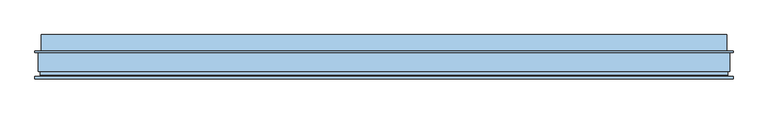
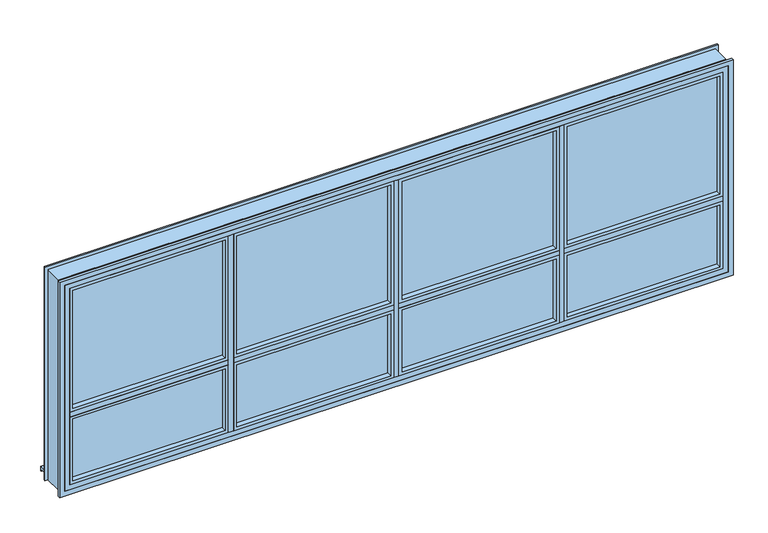
"""IFC4 building model written with IfcOpenShell, lengths in millimetres: window geometry, K-LINE ENSEMBLE COMPOSE NEUF KLT-8Z-4H2V : WD531_K-LINE ENSEMBLE COMPOSE NEUF KLT-8Z-4H2V."""

from ifc_helpers import new_model, si_unit, frame, origin, place, context, project, spatial, polyline, outline, extrude, faceted_brep, source, transform, mapped, element, save


def window_16f5b6b2(model_context):
    return source(origin(), model_context, "Body", "SolidModel", [
        extrude(outline(polyline([(-18.0, -155.0), (-18.0, -179.0), (-882.0, -179.0), (-882.0, -155.0), (-18.0, -155.0)])), frame((0.0, 0.0, 850.5), z_axis=(0.0, 0.0, 1.0), x_axis=(1.0, 0.0, 0.0)), (0.0, 0.0, 1.0), 381.5),
        extrude(outline(polyline([(1236.0, -14.0), (1236.0, -886.0), (846.5, -886.0), (846.5, -14.0), (1236.0, -14.0)]), holes=[polyline([(863.5, -31.0), (863.5, -869.0), (1219.0, -869.0), (1219.0, -31.0), (863.5, -31.0)])]), frame((0.0, -207.5, 0.0), z_axis=(0.0, 1.0, 0.0), x_axis=(0.0, 0.0, 1.0)), (0.0, 0.0, 1.0), 28.5),
        extrude(outline(polyline([(-18.0, -155.0), (-18.0, -179.0), (-882.0, -179.0), (-882.0, -155.0), (-18.0, -155.0)])), frame((0.0, 0.0, 1268.0), z_axis=(0.0, 0.0, 1.0), x_axis=(1.0, 0.0, 0.0)), (0.0, 0.0, 1.0), 705.0),
        extrude(outline(polyline([(1977.0, -14.0), (1977.0, -886.0), (1264.0, -886.0), (1264.0, -14.0), (1977.0, -14.0)]), holes=[polyline([(1281.0, -31.0), (1281.0, -869.0), (1960.0, -869.0), (1960.0, -31.0), (1281.0, -31.0)])]), frame((0.0, -207.5, 0.0), z_axis=(0.0, 1.0, 0.0), x_axis=(0.0, 0.0, 1.0)), (0.0, 0.0, 1.0), 28.5),
        extrude(outline(polyline([(-188.500001, 1241.0), (-188.500001, 1259.0), (-155.0, 1259.0), (-155.0, 1284.0), (-147.5, 1284.0), (-147.5, 1216.0), (-155.000001, 1216.0), (-155.000001, 1241.0), (-188.500001, 1241.0)])), frame((-866.0, 0.0, 0.0), z_axis=(1.0, 0.0, 0.0), x_axis=(0.0, 1.0, 0.0)), (0.0, 0.0, 1.0), 832.0),
        extrude(outline(polyline([(-14.0, -207.5), (-886.0, -207.5), (-886.0, -188.500001), (-14.0, -188.500001), (-14.0, -207.5)])), frame((0.0, 0.0, 1236.0), z_axis=(0.0, 0.0, 1.0), x_axis=(1.0, 0.0, 0.0)), (0.0, 0.0, 1.0), 28.0),
        extrude(outline(polyline([(-891.0, -155.0), (-891.0, -188.5), (-909.0, -188.5), (-909.0, -155.0), (-934.0, -155.0), (-934.0, -147.5), (-866.0, -147.5), (-866.0, -155.0), (-891.0, -155.0)])), frame((0.0, 0.0, 866.5), z_axis=(0.0, 0.0, 1.0), x_axis=(1.0, 0.0, 0.0)), (0.0, 0.0, 1.0), 1090.5),
        extrude(outline(polyline([(-914.0, -207.5), (-914.0, -188.5), (-886.0, -188.5), (-886.0, -207.5), (-914.0, -207.5)])), frame((0.0, 0.0, 846.5), z_axis=(0.0, 0.0, 1.0), x_axis=(1.0, 0.0, 0.0)), (0.0, 0.0, 1.0), 1130.5),
        extrude(outline(polyline([(882.0, -155.0), (882.0, -179.0), (18.0, -179.0), (18.0, -155.0), (882.0, -155.0)])), frame((0.0, 0.0, 850.5), z_axis=(0.0, 0.0, 1.0), x_axis=(1.0, 0.0, 0.0)), (0.0, 0.0, 1.0), 381.5),
        extrude(outline(polyline([(1236.0, 886.0), (1236.0, 14.0), (846.5, 14.0), (846.5, 886.0), (1236.0, 886.0)]), holes=[polyline([(863.5, 869.0), (863.5, 31.0), (1219.0, 31.0), (1219.0, 869.0), (863.5, 869.0)])]), frame((0.0, -207.5, 0.0), z_axis=(0.0, 1.0, 0.0), x_axis=(0.0, 0.0, 1.0)), (0.0, 0.0, 1.0), 28.5),
        extrude(outline(polyline([(882.0, -155.0), (882.0, -179.0), (18.0, -179.0), (18.0, -155.0), (882.0, -155.0)])), frame((0.0, 0.0, 1268.0), z_axis=(0.0, 0.0, 1.0), x_axis=(1.0, 0.0, 0.0)), (0.0, 0.0, 1.0), 705.0),
        extrude(outline(polyline([(1977.0, 886.0), (1977.0, 14.0), (1264.0, 14.0), (1264.0, 886.0), (1977.0, 886.0)]), holes=[polyline([(1281.0, 869.0), (1281.0, 31.0), (1960.0, 31.0), (1960.0, 869.0), (1281.0, 869.0)])]), frame((0.0, -207.5, 0.0), z_axis=(0.0, 1.0, 0.0), x_axis=(0.0, 0.0, 1.0)), (0.0, 0.0, 1.0), 28.5),
        extrude(outline(polyline([(-188.500001, 1241.0), (-188.500001, 1259.0), (-155.0, 1259.0), (-155.0, 1284.0), (-147.5, 1284.0), (-147.5, 1216.0), (-155.000001, 1216.0), (-155.000001, 1241.0), (-188.500001, 1241.0)])), frame((34.0, 0.0, 0.0), z_axis=(1.0, 0.0, 0.0), x_axis=(0.0, 1.0, 0.0)), (0.0, 0.0, 1.0), 832.0),
        extrude(outline(polyline([(886.0, -207.5), (14.0, -207.5), (14.0, -188.500001), (886.0, -188.500001), (886.0, -207.5)])), frame((0.0, 0.0, 1236.0), z_axis=(0.0, 0.0, 1.0), x_axis=(1.0, 0.0, 0.0)), (0.0, 0.0, 1.0), 28.0),
        extrude(outline(polyline([(9.0, -155.0), (9.0, -188.5), (-9.0, -188.5), (-9.0, -155.0), (-34.0, -155.0), (-34.0, -147.5), (34.0, -147.5), (34.0, -155.0), (9.0, -155.0)])), frame((0.0, 0.0, 866.5), z_axis=(0.0, 0.0, 1.0), x_axis=(1.0, 0.0, 0.0)), (0.0, 0.0, 1.0), 1090.5),
        extrude(outline(polyline([(-14.0, -207.5), (-14.0, -188.5), (14.0, -188.5), (14.0, -207.5), (-14.0, -207.5)])), frame((0.0, 0.0, 846.5), z_axis=(0.0, 0.0, 1.0), x_axis=(1.0, 0.0, 0.0)), (0.0, 0.0, 1.0), 1130.5),
        extrude(outline(polyline([(1773.0, -155.0), (1773.0, -179.0), (918.0, -179.0), (918.0, -155.0), (1773.0, -155.0)])), frame((0.0, 0.0, 850.5), z_axis=(0.0, 0.0, 1.0), x_axis=(1.0, 0.0, 0.0)), (0.0, 0.0, 1.0), 381.5),
        extrude(outline(polyline([(1236.0, 1777.0), (1236.0, 914.0), (846.5, 914.0), (846.5, 1777.0), (1236.0, 1777.0)]), holes=[polyline([(863.5, 1760.0), (863.5, 931.0), (1219.0, 931.0), (1219.0, 1760.0), (863.5, 1760.0)])]), frame((0.0, -207.5, 0.0), z_axis=(0.0, 1.0, 0.0), x_axis=(0.0, 0.0, 1.0)), (0.0, 0.0, 1.0), 28.5),
        extrude(outline(polyline([(-918.0, -155.0), (-918.0, -179.0), (-1773.0, -179.0), (-1773.0, -155.0), (-918.0, -155.0)])), frame((0.0, 0.0, 850.5), z_axis=(0.0, 0.0, 1.0), x_axis=(1.0, 0.0, 0.0)), (0.0, 0.0, 1.0), 381.5),
        extrude(outline(polyline([(1236.0, -914.0), (1236.0, -1777.0), (846.5, -1777.0), (846.5, -914.0), (1236.0, -914.0)]), holes=[polyline([(863.5, -931.0), (863.5, -1760.0), (1219.0, -1760.0), (1219.0, -931.0), (863.5, -931.0)])]), frame((0.0, -207.5, 0.0), z_axis=(0.0, 1.0, 0.0), x_axis=(0.0, 0.0, 1.0)), (0.0, 0.0, 1.0), 28.5),
        extrude(outline(polyline([(-188.500001, 1241.0), (-188.500001, 1259.0), (-155.0, 1259.0), (-155.0, 1284.0), (-147.5, 1284.0), (-147.5, 1216.0), (-155.000001, 1216.0), (-155.000001, 1241.0), (-188.500001, 1241.0)])), frame((-1757.0, 0.0, 0.0), z_axis=(1.0, 0.0, 0.0), x_axis=(0.0, 1.0, 0.0)), (0.0, 0.0, 1.0), 823.0),
        extrude(outline(polyline([(-914.0, -207.5), (-1777.0, -207.5), (-1777.0, -188.500001), (-914.0, -188.500001), (-914.0, -207.5)])), frame((0.0, 0.0, 1236.0), z_axis=(0.0, 0.0, 1.0), x_axis=(1.0, 0.0, 0.0)), (0.0, 0.0, 1.0), 28.0),
        extrude(outline(polyline([(-188.500001, 1241.0), (-188.500001, 1259.0), (-155.0, 1259.0), (-155.0, 1284.0), (-147.5, 1284.0), (-147.5, 1216.0), (-155.000001, 1216.0), (-155.000001, 1241.0), (-188.500001, 1241.0)])), frame((934.0, 0.0, 0.0), z_axis=(1.0, 0.0, 0.0), x_axis=(0.0, 1.0, 0.0)), (0.0, 0.0, 1.0), 823.0),
        extrude(outline(polyline([(1777.0, -207.5), (914.0, -207.5), (914.0, -188.500001), (1777.0, -188.500001), (1777.0, -207.5)])), frame((0.0, 0.0, 1236.0), z_axis=(0.0, 0.0, 1.0), x_axis=(1.0, 0.0, 0.0)), (0.0, 0.0, 1.0), 28.0),
        extrude(outline(polyline([(1773.0, -155.0), (1773.0, -179.0), (918.0, -179.0), (918.0, -155.0), (1773.0, -155.0)])), frame((0.0, 0.0, 1268.0), z_axis=(0.0, 0.0, 1.0), x_axis=(1.0, 0.0, 0.0)), (0.0, 0.0, 1.0), 705.0),
        extrude(outline(polyline([(1977.0, 1777.0), (1977.0, 914.0), (1264.0, 914.0), (1264.0, 1777.0), (1977.0, 1777.0)]), holes=[polyline([(1281.0, 1760.0), (1281.0, 931.0), (1960.0, 931.0), (1960.0, 1760.0), (1281.0, 1760.0)])]), frame((0.0, -207.5, 0.0), z_axis=(0.0, 1.0, 0.0), x_axis=(0.0, 0.0, 1.0)), (0.0, 0.0, 1.0), 28.5),
        extrude(outline(polyline([(-918.0, -155.0), (-918.0, -179.0), (-1773.0, -179.0), (-1773.0, -155.0), (-918.0, -155.0)])), frame((0.0, 0.0, 1268.0), z_axis=(0.0, 0.0, 1.0), x_axis=(1.0, 0.0, 0.0)), (0.0, 0.0, 1.0), 705.0),
        extrude(outline(polyline([(1977.0, -914.0), (1977.0, -1777.0), (1264.0, -1777.0), (1264.0, -914.0), (1977.0, -914.0)]), holes=[polyline([(1281.0, -931.0), (1281.0, -1760.0), (1960.0, -1760.0), (1960.0, -931.0), (1281.0, -931.0)])]), frame((0.0, -207.5, 0.0), z_axis=(0.0, 1.0, 0.0), x_axis=(0.0, 0.0, 1.0)), (0.0, 0.0, 1.0), 28.5),
        extrude(outline(polyline([(909.0, -155.0), (909.0, -188.5), (891.0, -188.5), (891.0, -155.0), (866.0, -155.0), (866.0, -147.5), (934.0, -147.5), (934.0, -155.0), (909.0, -155.0)])), frame((0.0, 0.0, 866.5), z_axis=(0.0, 0.0, 1.0), x_axis=(1.0, 0.0, 0.0)), (0.0, 0.0, 1.0), 1090.5),
        extrude(outline(polyline([(886.0, -207.5), (886.0, -188.5), (914.0, -188.5), (914.0, -207.5), (886.0, -207.5)])), frame((0.0, 0.0, 846.5), z_axis=(0.0, 0.0, 1.0), x_axis=(1.0, 0.0, 0.0)), (0.0, 0.0, 1.0), 1130.5),
        extrude(outline(polyline([(2032.0, 1832.0), (2032.0, -1832.0), (791.5, -1832.0), (791.5, 1832.0), (2032.0, 1832.0)]), holes=[polyline([(818.4999998, 1805.0000002), (818.4999998, -1805.0000002), (2005.0000002, -1805.0000002), (2005.0000002, 1805.0000002), (818.4999998, 1805.0000002)])]), frame((0.0, -207.5, 0.0), z_axis=(0.0, 1.0, 0.0), x_axis=(0.0, 0.0, 1.0)), (0.0, 0.0, 1.0), 12.5),
        extrude(outline(polyline([(2005.0000002, 1805.0000002), (2005.0000002, -1805.0000002), (818.4999998, -1805.0000002), (818.4999998, 1805.0000002), (2005.0000002, 1805.0000002)]), holes=[polyline([(846.5, 1777.0), (846.5, -1777.0), (1977.0, -1777.0), (1977.0, 1777.0), (846.5, 1777.0)])]), frame((0.0, -207.5, 0.0), z_axis=(0.0, 1.0, 0.0), x_axis=(0.0, 0.0, 1.0)), (0.0, 0.0, 1.0), 19.0),
        faceted_brep([(1756.999999, -154.9965859, 1956.999999), (1756.999999, -147.4965859, 1956.999999), (1756.999999, -147.4965859, 866.500001), (1756.999999, -154.9965859, 866.500001), (1805.0000002, -147.4965859, 818.4999998), (-1805.0000002, -147.4965859, 818.4999998), (-1805.0000002, -147.4965859, 2005.0000002), (1805.0000002, -147.4965859, 2005.0000002), (-1756.999999, -147.4965859, 1956.999999), (-1756.999999, -147.4965859, 866.500001), (-1756.999999, -154.9965859, 866.500001), (1782.0, -154.9965859, 1982.0), (-1782.0, -154.9965859, 1982.0), (-1782.0, -154.9965859, 841.5), (1782.0, -154.9965859, 841.5), (-1756.999999, -154.9965859, 1956.999999), (1782.0, -188.5, 1982.0), (1782.0, -188.5, 841.5), (-1782.0, -188.5, 841.5), (1805.0000002, -188.5, 2005.0000002), (-1805.0000002, -188.5, 2005.0000002), (-1805.0000002, -188.5, 818.4999998), (1805.0000002, -188.5, 818.4999998), (-1782.0, -188.5, 1982.0)], [[[0, 1, 2, 3]], [[4, 5, 6, 7], [1, 8, 9, 2]], [[3, 2, 9, 10]], [[11, 12, 13, 14], [3, 10, 15, 0]], [[16, 11, 14, 17]], [[17, 14, 13, 18]], [[19, 20, 21, 22], [17, 18, 23, 16]], [[7, 19, 22, 4]], [[4, 22, 21, 5]], [[10, 9, 8, 15]], [[18, 13, 12, 23]], [[5, 21, 20, 6]], [[15, 8, 1, 0]], [[23, 12, 11, 16]], [[6, 20, 19, 7]]]),
        faceted_brep([(-1815.0, -68.0, 805.0), (-1832.0, -68.0, 805.0), (-1832.0, -60.0, 805.0), (-1800.0, -60.0, 805.0), (-1800.0, -147.4965859, 805.0), (-1805.0, -147.4965859, 805.0), (-1805.0, -166.4965859, 805.0), (-1815.0, -166.4965859, 805.0), (-1815.0, -68.0, 2015.0), (1815.0, -68.0, 2015.0), (1815.0, -68.0, 805.0), (1832.0, -68.0, 805.0), (1832.0, -68.0, 2032.0), (-1832.0, -68.0, 2032.0), (-1832.0, -60.0, 2032.0), (1832.0, -60.0, 2032.0), (1832.0, -60.0, 805.0), (1800.0, -60.0, 805.0), (1800.0, -60.0, 2000.0), (-1800.0, -60.0, 2000.0), (-1800.0, -147.4965859, 2000.0), (1800.0, -147.4965859, 2000.0), (1800.0, -147.4965859, 805.0), (1805.0, -147.4965859, 805.0), (1805.0, -147.4965859, 2005.0), (-1805.0, -147.4965859, 2005.0), (-1805.0, -166.4965859, 2005.0), (1805.0, -166.4965859, 2005.0), (1805.0, -166.4965859, 805.0), (1815.0, -166.4965859, 805.0), (1815.0, -166.4965859, 2015.0), (-1815.0, -166.4965859, 2015.0)], [[[0, 1, 2, 3, 4, 5, 6, 7]], [[1, 0, 8, 9, 10, 11, 12, 13]], [[2, 1, 13, 14]], [[3, 2, 14, 15, 16, 17, 18, 19]], [[5, 4, 20, 21, 22, 23, 24, 25]], [[6, 5, 25, 26]], [[7, 6, 26, 27, 28, 29, 30, 31]], [[0, 7, 31, 8]], [[15, 12, 11, 16]], [[10, 29, 28, 23, 22, 17, 16, 11]], [[27, 24, 23, 28]], [[9, 30, 29, 10]], [[14, 13, 12, 15]], [[26, 25, 24, 27]], [[8, 31, 30, 9]], [[4, 3, 19, 20]], [[21, 18, 17, 22]], [[20, 19, 18, 21]]]),
        extrude(outline(polyline([(-147.4965859, 825.311129), (25.8038196, 819.2593455), (25.8038196, 794.3604516), (21.4038196, 794.3604516), (21.4038196, 805.0000004), (-161.2965876, 805.0000004), (-161.2965876, 818.5), (-147.4965859, 818.5), (-147.4965859, 825.311129)])), frame((-1800.0, 0.0, 0.0), z_axis=(1.0, 0.0, 0.0), x_axis=(0.0, 1.0, 0.0)), (0.0, 0.0, 1.0), 3600.0),
    ])


if __name__ == "__main__":
    model = new_model("IFC4")
    model_context = context("Model", 3, world=origin())
    ifc_project = project(units=[si_unit("LENGTHUNIT", "METRE", prefix="MILLI")], contexts=[model_context])
    site = spatial("IfcSite", under=ifc_project)
    building = spatial("IfcBuilding", under=site)
    placement = place(None, origin())
    window_shape = window_16f5b6b2(model_context)
    element("IfcWindow", 1, ObjectType="K-LINE ENSEMBLE COMPOSE NEUF KLT-8Z-4H2V : WD531_K-LINE ENSEMBLE COMPOSE NEUF KLT-8Z-4H2V", at=placement, inside=building, context=model_context, shape_type="MappedRepresentation", body=[
        mapped(window_shape, transform((0.0, 0.0, 0.0), x_axis=(1.0, 0.0, 0.0), y_axis=(0.0, 1.0, 0.0), z_axis=(0.0, 0.0, 1.0))),
    ])
    save(model, "model.ifc")

# Revit data of these elements
# Type "K-LINE ENSEMBLE COMPOSE NEUF KLT-8Z-4H2V : WD531_K-LINE ENSEMBLE COMPOSE NEUF KLT-8Z-4H2V"
#   Type Mark = "AW"
#   Vitrage secondaire = ""
#   Vitrage principal = ""
#   URL = "https://pro.k-line.fr/bandes-ensembles-composes-kl-t.aspx"
#   Type de pose = "ITI"
#   Transmission lumineuse TLw = "67%"
#   SAV = "https://sav.k-line.fr/"
#   Product data url = "https://www.bimobject.com/k-line/product/klt-8zec2h4v"
#   Outil de thermo-luminosité = "http://www.pro.k-line.fr/calculateur-presentation.aspx"
#   Occultation = "Non"
#   Numéro de série = "K.........."
#   Keynote = "08520"
#   Neuf / Réno / Multi support = "Neuf"
#   Mortaise et grille d'entrée d'air = ""
#   Model = "KL-T Châssis Ensemble composé 8 Zones"
#   Matériaux = "Aluminium et verre"
#   Information renfort d'inertie = "Les renforts intérieurs ne sont compatible avec des ouvrants que sur des profils de 200mm de largeur"
#   Garanties = "https://pro.k-line.fr/pdf/attestations/Garanties_Legales_KLINE.pdf"
#   Famille de produit = "KL-City"
#   Manufacturer = "K.LINE"
#   Entretien = "https://pro.k-line.fr/pdf/ficheproduit/laq_fiche_entretien.pdf"
#   Entreprise de pose = ""
#   Doublages disponibles = "80,100,110,120,130,140,160,180 et 200 mm"
#   Description = "Fenêtre Alu"
#   Analytic Construction = "<Aucun>"
#   Composition analytique de base = "Châssis 1250x1480 - Vitrage 4/WE Argon 16/TBE 4 - Finition Black"
#   Classement AEV = "A*4 E*7B V*A3"
#   Classe COV = "A+"
#   Avis technique = "https://pro.k-line.fr/attestations-avis-technique.aspx"
#   Affaiblissement acoustique R(A,tr) = "30dB"
#   Val décal appui = 100 mm
#   Transmission thermique Uw = 1.4000 W/(m²·K)
#   Surface = 4.32 m²
#   Profondeur symbole d'ouverture = 150 mm
#   Position doublage = 0 mm
#   Lg traverse 4 = 909 mm
#   Lg traverse 3 = 918 mm
#   Lg traverse 2 = 918 mm
#   Lg traverse 1 = 909 mm
#   Largeur zone 4 = 900 mm
#   Largeur zone 3 = 900 mm
#   Largeur zone 2 = 900 mm
#   Largeur zone 1 = 900 mm
#   Largeur ouvrant 4 = 839 mm
#   Largeur ouvrant 3 = 848 mm
#   Largeur ouvrant 2 = 848 mm
#   Largeur ouvrant 1 = 839 mm
#   Rough Width [instance default] = 3600 mm
#   Largeur Traverse intermédiaire : 68,85,100,150,175 et 200 = 68 mm
#   Largeur Montant intermédiaire : 68,85,100,150,175 et 200 = 68 mm
#   Hauteur zone 5 = 750 mm
#   Hauteur zone 1 = 450 mm
#   Hauteur ouvrant 4/5/6 = 689 mm
#   Hauteur ouvrant 1/2/3 = 365.5 mm
#   Hauteur de poignée = 318 mm
#   Rough Height [instance default] = 1200 mm
#   Height = 1200 mm
#   Hauteur de l'appui par défaut = 800 mm
#   H profil = 1090.5 mm
#   Width = 3600 mm
#   Facteur solaire ScW (Hiver) = 0.53
#   Décalage appui = 180 mm
#   Décal appui = 40 mm
#   Doublage + ratrapage = 140 mm
#   Doublage = 140 mm
#   Centre zone 5/6/7/8 = 344.5 mm
#   Centre zone 1/2/3/4 = 182.75 mm
#   Centre Ouvrant 4/8 = 419.5 mm
#   Centre Ouvrant 3/7 = 450 mm
#   Centre Ouvrant 2/6 = 450 mm
#   Centre Ouvrant 1/5 = 419.5 mm
#   Angle symbole d'ouverture = 15.00°
#   Symbole d'ouverture = yes
#   Renfort saillant Intérieur = no
#   Renfort saillant Extérieur = no
#   Renfort Int saillant de 67.5 = no
#   Renfort Int saillant de 107.5 = yes
#   Renfort Ext saillant de 67.5 = no
#   Renfort Ext saillant de 107.5 = yes
#   Rattrapage doublage = no
#   Option appui sans aile intérieure = no
#   Finition Métal = yes
#   Finition Black = no
#   Rattrapage avec aile = no
#   Appui Non-Déporté = no
#   Appui Déporté = yes
#   Vitrage = Verre
#   Type d'ouvrant zone 8 = element 2302654
#   Type d'ouvrant zone 7 = element 2302654
#   Type d'ouvrant zone 6 = element 2302654
#   Type d'ouvrant zone 5 = element 2302654
#   Type d'ouvrant zone 4 = element 2302654
#   Type d'ouvrant zone 3 = element 2302654
#   Type d'ouvrant zone 2 = element 2302654
#   Type d'ouvrant zone 1 = element 2302654
#   Couleur panneau opaque Int = K.Line Intemporel Blanc satiné (9016 S) - KQ
#   Couleur panneau opaque Ext = K.Line Tendance Grège (9007 T) - RQ
#   Couleur châssis Int = K.Line Intemporel Blanc satiné (9016 S) - KQ
#   Couleur châssis Ext = K.Line Tendance Grège (9007 T) - RQ
#   Couleur Accessoire Int = K.Line Accessoire Blanc - KQ
#   Wall Closure = (empty or 0)
# Element 1 (IfcWindow, "K-LINE ENSEMBLE COMPOSE NEUF KLT-8Z-4H2V : WD531_K-LINE ENSEMBLE COMPOSE NEUF KLT-8Z-4H2V")
#   Materials on its faces: "K.Line Intemporel Blanc satiné (9016 S) - KQ", "K.Line Tendance Grège (9007 T) - RQ", "Verre"
# Materials
#   "Verre": class "Verre", colour RGB 92 99 177, transparency 0.7, Description = "AL. WINDOW(TYP.)", Cost = 0
#   "K.Line Intemporel Blanc satiné (9016 S) - KQ": class "Metal", colour RGB 247 246 246, transparency 0, Description = "Aluminum 6061", Cost = 0
#   "K.Line Tendance Grège (9007 T) - RQ": class "Metal", colour RGB 135 133 129, transparency 0, Description = "Aluminum 6061", Cost = 0
#   "K.Line Accessoire Blanc - KQ": class "Metal", colour RGB 247 246 246, transparency 0, Description = "Aluminum 6061", Cost = 0
